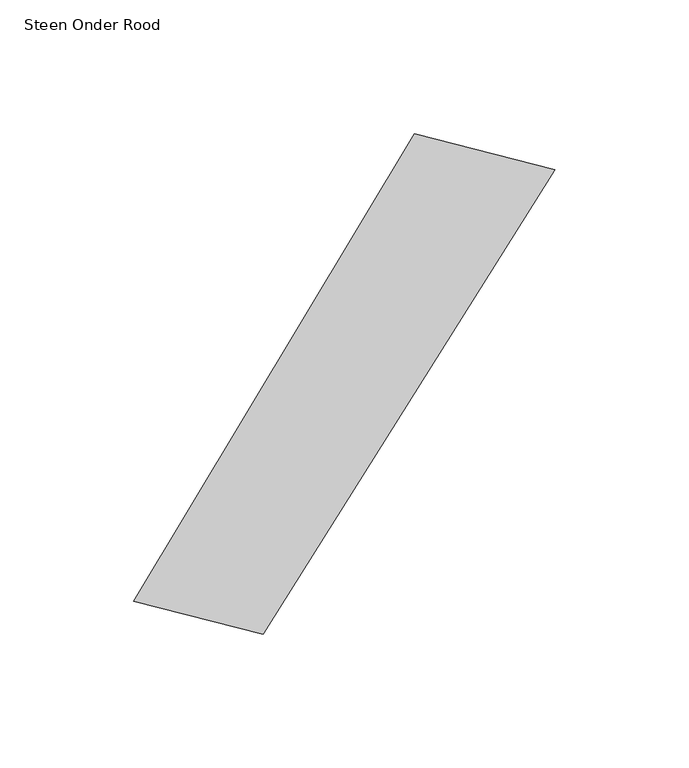
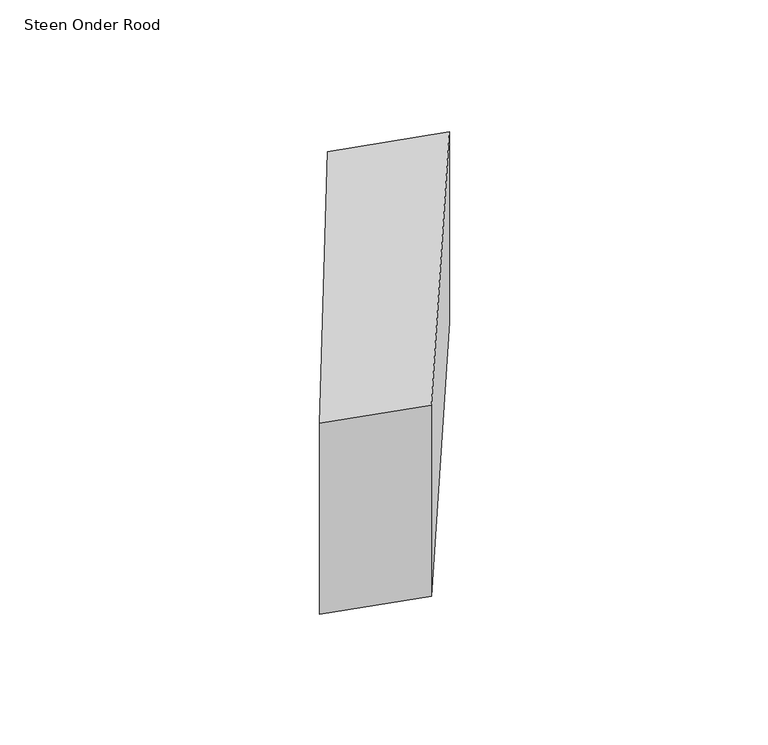
"""IFC4 building model written with IfcOpenShell, lengths in millimetres: proxy geometry, 00_GMA_steen_versie_4 : Steen Onder Rood."""

from ifc_helpers import new_model, si_unit, origin, origin_with_axes, place, context, project, spatial, polyline, outline, extrude, source, transform, mapped, element, save


def steen_onder_rood_8f19e249(model_context):
    return source(origin(), model_context, "Body", "SweptSolid", [
        extrude(outline(polyline([(153.9671513, 154.5404053), (44.7869952, -19.1132829), (-3.6641694, -6.7648155), (101.296672, 167.9379986), (153.9671513, 154.5404053)])), origin_with_axes(), (0.0, 0.0, 1.0), 100.0),
    ])


if __name__ == "__main__":
    model = new_model("IFC4")
    model_context = context("Model", 3, world=origin())
    ifc_project = project(units=[si_unit("LENGTHUNIT", "METRE", prefix="MILLI")], contexts=[model_context])
    site = spatial("IfcSite", under=ifc_project)
    building = spatial("IfcBuilding", under=site)
    placement = place(None, origin())
    steen_onder_rood_shape = steen_onder_rood_8f19e249(model_context)
    element("IfcBuildingElementProxy", 1, Name="00_GMA_steen_versie_4 : Steen Onder Rood", ObjectType="00_GMA_steen_versie_4 : Steen Onder Rood", at=placement, inside=building, context=model_context, shape_type="MappedRepresentation", body=[
        mapped(steen_onder_rood_shape, transform((0.0, 0.0, 0.0), x_axis=(1.0, 0.0, 0.0), y_axis=(0.0, 1.0, 0.0), z_axis=(0.0, 0.0, 1.0))),
    ])
    save(model, "model.ifc")

# Revit data of these elements
# Type "00_GMA_steen_versie_4 : Steen Onder Rood"
#   StootVoegHalfBoven [instance default] = 5 mm
#   StootVoegHalf [instance default] = 5 mm
#   StootVoegBreedteOnder = 10 mm
#   StootVoegBreedteBoven = 10 mm
#   Steendikte = 100 mm
#   LintVoegOnderHalf = 0 mm
#   LintVoegOnder = 0 mm
#   LintVoegBovenHalf = 5 mm
#   LintVoegBoven = 10 mm
#   materiaal = 21_steen_rood
#   MateriaalVoeg = none
#   Default Elevation = 0
# Element 1 (IfcBuildingElementProxy, "00_GMA_steen_versie_4 : Steen Onder Rood")
#   Materials on its faces: "21_steen_rood"
# Materials
#   "21_steen_rood": class "Unassigned", colour RGB 213 111 43, transparency 0, Cost = 0
